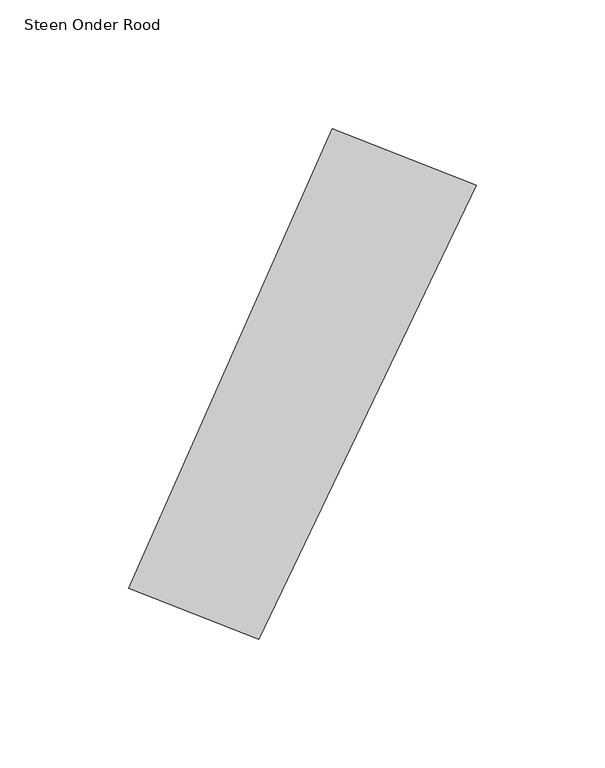
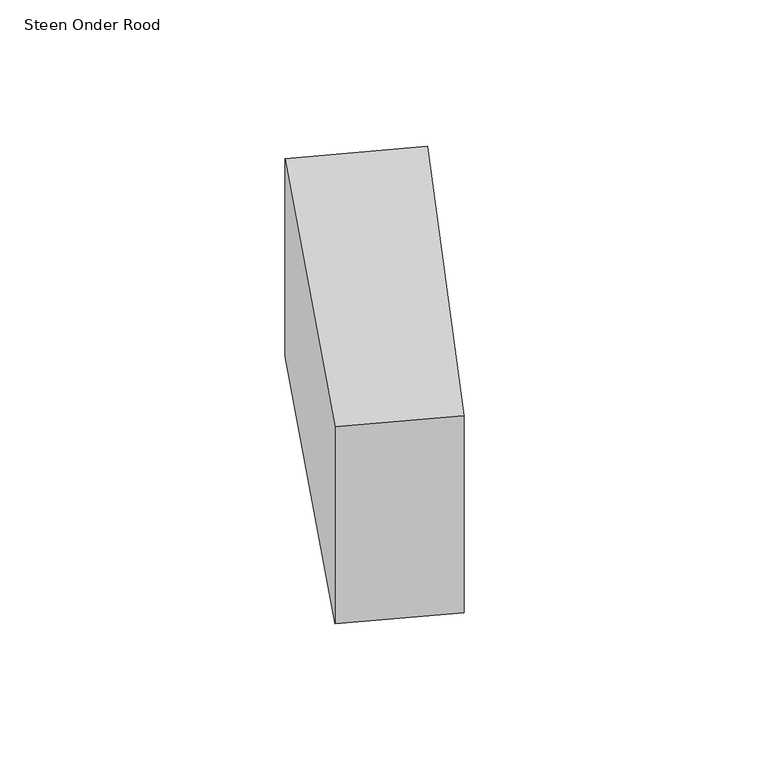
"""IFC4 building model written with IfcOpenShell, lengths in millimetres: proxy geometry, 00_GMA_steen_versie_4 : Steen Onder Rood."""

from ifc_helpers import new_model, si_unit, origin, origin_with_axes, place, context, project, spatial, polyline, outline, extrude, source, transform, mapped, element, save


def steen_onder_rood_81b8b642(model_context):
    return source(origin(), model_context, "Body", "SweptSolid", [
        extrude(outline(polyline([(141.9885303, 156.3667337), (57.6485421, -20.0413331), (7.0756111, -0.2498175), (86.1042269, 178.2290117), (141.9885303, 156.3667337)])), origin_with_axes(), (0.0, 0.0, 1.0), 100.0),
    ])


if __name__ == "__main__":
    model = new_model("IFC4")
    model_context = context("Model", 3, world=origin())
    ifc_project = project(units=[si_unit("LENGTHUNIT", "METRE", prefix="MILLI")], contexts=[model_context])
    site = spatial("IfcSite", under=ifc_project)
    building = spatial("IfcBuilding", under=site)
    placement = place(None, origin())
    steen_onder_rood_shape = steen_onder_rood_81b8b642(model_context)
    element("IfcBuildingElementProxy", 1, Name="00_GMA_steen_versie_4 : Steen Onder Rood", ObjectType="00_GMA_steen_versie_4 : Steen Onder Rood", at=placement, inside=building, context=model_context, shape_type="MappedRepresentation", body=[
        mapped(steen_onder_rood_shape, transform((0.0, 0.0, 0.0), x_axis=(1.0, 0.0, 0.0), y_axis=(0.0, 1.0, 0.0), z_axis=(0.0, 0.0, 1.0))),
    ])
    save(model, "model.ifc")

# Revit data of these elements
# Type "00_GMA_steen_versie_4 : Steen Onder Rood"
#   StootVoegHalfBoven [instance default] = 5 mm
#   StootVoegHalf [instance default] = 5 mm
#   StootVoegBreedteOnder = 10 mm
#   StootVoegBreedteBoven = 10 mm
#   Steendikte = 100 mm
#   LintVoegOnderHalf = 0 mm
#   LintVoegOnder = 0 mm
#   LintVoegBovenHalf = 5 mm
#   LintVoegBoven = 10 mm
#   materiaal = 21_steen_rood
#   MateriaalVoeg = none
#   Default Elevation = 0
# Element 1 (IfcBuildingElementProxy, "00_GMA_steen_versie_4 : Steen Onder Rood")
#   Materials on its faces: "21_steen_rood"
# Materials
#   "21_steen_rood": class "Unassigned", colour RGB 213 111 43, transparency 0, Cost = 0
